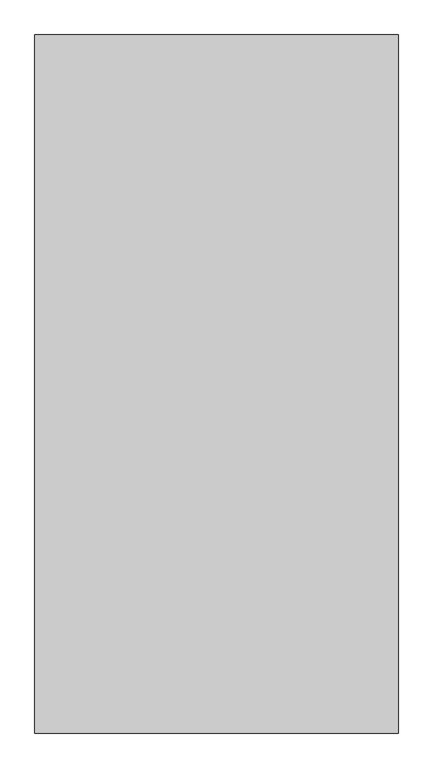
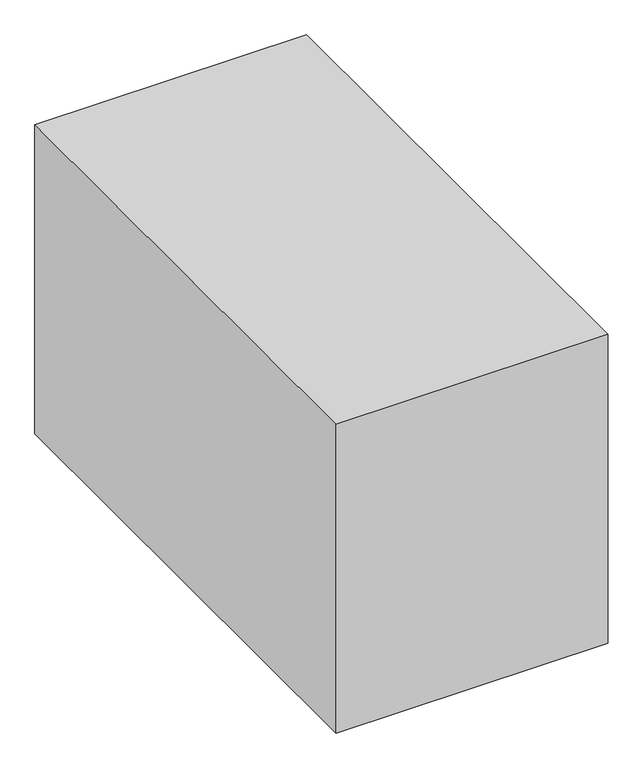
"""IFC4 building model written with IfcOpenShell, lengths in millimetres: proxy geometry, Space Planning Box_hec : Space Planning Box_hec."""

import ifcopenshell
import ifcopenshell.guid

model = None  # the IFC model being written
_history = None  # IfcOwnerHistory: only IFC2X3 demands one
_inside = {}  # id of a spatial element -> (the spatial element, [elements in it])
_under = {}  # id of a project, library or spatial element -> (it, [spatial elements below it])
_declared = {}  # id of a project -> (the project, [libraries it declares])
_typed = {}  # id of a type object -> (the type object, [elements of that type])
_made_of = {}  # id of a material, layer set ... -> (it, [elements and type objects made of it])


def new_model(schema):
    """Start an empty IFC model of exactly this schema.

    Asked for "IFC4X3", IfcOpenShell would pick the latest addendum, in which some entities
    have other attributes; the version numbers below select the first issue.
    IFC2X3 requires an IfcOwnerHistory on every rooted entity: one is made here for all.
    """
    global model, _history
    if schema == "IFC4X3":
        model = ifcopenshell.file(schema_version=(4, 3, 0, 0))
    else:
        model = ifcopenshell.file(schema=schema)
    _inside.clear()
    _under.clear()
    _declared.clear()
    _typed.clear()
    _made_of.clear()
    _history = None
    if model.schema == "IFC2X3":
        org = make("IfcOrganization", Name="unknown")
        user = make(
            "IfcPersonAndOrganization",
            ThePerson=make("IfcPerson", FamilyName="unknown"),
            TheOrganization=org,
        )
        app = make(
            "IfcApplication",
            ApplicationDeveloper=org,
            Version="unknown",
            ApplicationFullName="unknown",
            ApplicationIdentifier="unknown",
        )
        _history = make(
            "IfcOwnerHistory",
            OwningUser=user,
            OwningApplication=app,
            ChangeAction="ADDED",
            CreationDate=0,
        )
    return model


def make(cls, **values):
    """One entity of the class cls with the attributes given. An attribute that is None is left unset."""
    return model.create_entity(
        cls, **{name: value for name, value in values.items() if value is not None}
    )


def rooted(cls, **values):
    """An entity with a GlobalId (a new one), such as an element, a storey or a relation."""
    return make(cls, GlobalId=ifcopenshell.guid.new(), OwnerHistory=_history, **values)


def si_unit(unit_type, name, prefix=None):
    """IfcSIUnit, for example si_unit("LENGTHUNIT", "METRE", prefix="MILLI")."""
    return make("IfcSIUnit", UnitType=unit_type, Prefix=prefix, Name=name)


def assignment(units):
    """IfcUnitAssignment: the units of a project."""
    return None if units is None else make("IfcUnitAssignment", Units=units)


def point(xyz):
    """IfcCartesianPoint."""
    return None if xyz is None else make("IfcCartesianPoint", Coordinates=xyz)


def direction(xyz):
    """IfcDirection."""
    return None if xyz is None else make("IfcDirection", DirectionRatios=xyz)


def frame(location, z_axis=None, x_axis=None):
    """IfcAxis2Placement3D, a coordinate frame: its origin and axes. An axis left out is left unset."""
    return make(
        "IfcAxis2Placement3D",
        Location=point(location),
        Axis=direction(z_axis),
        RefDirection=direction(x_axis),
    )


def origin():
    """The frame at (0, 0, 0) with its axes left unset."""
    return frame((0.0, 0.0, 0.0))


def origin_with_axes():
    """The frame at (0, 0, 0) with the z axis (0, 0, 1) and the x axis (1, 0, 0) written out."""
    return frame((0.0, 0.0, 0.0), z_axis=(0.0, 0.0, 1.0), x_axis=(1.0, 0.0, 0.0))


def place(relative_to, where):
    """IfcLocalPlacement: puts the frame where relative to a parent placement (None: the world)."""
    return make(
        "IfcLocalPlacement", PlacementRelTo=relative_to, RelativePlacement=where
    )


def context(
    kind, dimensions, precision=None, world=None, true_north=None, identifier=None
):
    """IfcGeometricRepresentationContext, for example the 3D "Model" context."""
    return make(
        "IfcGeometricRepresentationContext",
        ContextIdentifier=identifier,
        ContextType=kind,
        CoordinateSpaceDimension=dimensions,
        Precision=precision,
        WorldCoordinateSystem=world,
        TrueNorth=true_north,
    )


def project(units=None, contexts=None):
    """IfcProject with its units and contexts."""
    return rooted(
        "IfcProject",
        Name="project",
        RepresentationContexts=contexts,
        UnitsInContext=assignment(units),
    )


def spatial(cls, under=None, at=None, **own):
    """A site, building, storey or space (cls), placed at a placement, below another one or the project."""
    s = rooted(cls, ObjectPlacement=at, **own)
    if under is not None:
        _under.setdefault(under.id(), (under, []))[1].append(s)
    return s


def polyline(points):
    """IfcPolyline through the points."""
    return make("IfcPolyline", Points=[point(p) for p in points])


def outline(outer, holes=None, kind="AREA"):
    """IfcArbitraryClosedProfileDef: a profile drawn as a closed curve; with holes, ...WithVoids."""
    if holes is None:
        return make("IfcArbitraryClosedProfileDef", ProfileType=kind, OuterCurve=outer)
    return make(
        "IfcArbitraryProfileDefWithVoids",
        ProfileType=kind,
        OuterCurve=outer,
        InnerCurves=holes,
    )


def extrude(swept, where, along, depth):
    """IfcExtrudedAreaSolid: the profile swept, set in the frame where, extruded along a direction by depth."""
    return make(
        "IfcExtrudedAreaSolid",
        SweptArea=swept,
        Position=where,
        ExtrudedDirection=direction(along),
        Depth=depth,
    )


def shape(context_of_items, identifier, shape_type, items):
    """IfcShapeRepresentation: the items that make up one representation, for example the "Body"."""
    return make(
        "IfcShapeRepresentation",
        ContextOfItems=context_of_items,
        RepresentationIdentifier=identifier,
        RepresentationType=shape_type,
        Items=items,
    )


def source(mapping_origin, context_of_items, identifier, shape_type, items):
    """IfcRepresentationMap: a shape defined once, which mapped items show again and again."""
    return make(
        "IfcRepresentationMap",
        MappingOrigin=mapping_origin,
        MappedRepresentation=shape(context_of_items, identifier, shape_type, items),
    )


def transform(
    local_origin,
    x_axis=None,
    y_axis=None,
    z_axis=None,
    scale=None,
    scale2=None,
    scale3=None,
    uniform=True,
):
    """IfcCartesianTransformationOperator3D, or its non-uniform kind. x_axis, y_axis, z_axis: its Axis1, 2, 3."""
    if uniform:
        return make(
            "IfcCartesianTransformationOperator3D",
            Axis1=direction(x_axis),
            Axis2=direction(y_axis),
            LocalOrigin=point(local_origin),
            Scale=scale,
            Axis3=direction(z_axis),
        )
    return make(
        "IfcCartesianTransformationOperator3DnonUniform",
        Axis1=direction(x_axis),
        Axis2=direction(y_axis),
        LocalOrigin=point(local_origin),
        Scale=scale,
        Axis3=direction(z_axis),
        Scale2=scale2,
        Scale3=scale3,
    )


def mapped(mapping_source, mapping_target):
    """IfcMappedItem: shows the shape of a source again, moved by a transform."""
    return make(
        "IfcMappedItem", MappingSource=mapping_source, MappingTarget=mapping_target
    )


def made_of(thing, what):
    """Note that an element or type object is made of a material, layer set ...; save() writes the relation."""
    if what is not None:
        _made_of.setdefault(what.id(), (what, []))[1].append(thing)
    return thing


def element(
    cls,
    number,
    at=None,
    inside=None,
    cuts=None,
    type_object=None,
    material=None,
    context=None,
    identifier="Body",
    shape_type=None,
    held_by="IfcProductDefinitionShape",
    body=None,
    shapes=None,
    **own,
):
    """One element of the class cls, such as IfcWall. Its Tag is "e" and its number.

    at: its placement. inside: the storey or other place that contains it. cuts: it is an
    opening in that element (IfcRelVoidsElement). A single representation is given by context,
    identifier, shape_type and body (its items); several are given by shapes. held_by: the class
    of the entity that holds the representations. save() writes the other relations.
    """
    e = rooted(cls, Tag="e%d" % number, ObjectPlacement=at, **own)
    if body is not None:
        shapes = [shape(context, identifier, shape_type, body)]
    if shapes is not None:
        e.Representation = make(held_by, Representations=shapes)
    if inside is not None:
        _inside.setdefault(inside.id(), (inside, []))[1].append(e)
    if cuts is not None:
        rooted(
            "IfcRelVoidsElement", RelatingBuildingElement=cuts, RelatedOpeningElement=e
        )
    if type_object is not None:
        _typed.setdefault(type_object.id(), (type_object, []))[1].append(e)
    return made_of(e, material)


def aggregate(whole, parts):
    """IfcRelAggregates: a whole, such as a stair, and the parts it consists of."""
    return rooted("IfcRelAggregates", RelatingObject=whole, RelatedObjects=parts)


def save(model, path):
    """Write the relations noted so far, then the file.

    IfcRelAggregates (storeys below a building ...), IfcRelContainedInSpatialStructure (elements
    in a storey), IfcRelDefinesByType, IfcRelAssociatesMaterial and IfcRelDeclares: one each for
    every whole, place, type object, material and project.
    """
    for whole, parts in _under.values():
        aggregate(whole, parts)
    for where, things in _inside.values():
        rooted(
            "IfcRelContainedInSpatialStructure",
            RelatedElements=things,
            RelatingStructure=where,
        )
    for kind, things in _typed.values():
        rooted("IfcRelDefinesByType", RelatedObjects=things, RelatingType=kind)
    for what, things in _made_of.values():
        rooted("IfcRelAssociatesMaterial", RelatedObjects=things, RelatingMaterial=what)
    for by, libraries in _declared.values():
        rooted("IfcRelDeclares", RelatingContext=by, RelatedDefinitions=libraries)
    model.write(path)


def generic_models_7902148a(model_context):
    return source(origin(), model_context, "Body", "SweptSolid", [
        extrude(outline(polyline([(2500.0, 4800.0), (2500.0, -4800.0), (-2500.0, -4800.0), (-2500.0, 4800.0), (2500.0, 4800.0)])), origin_with_axes(), (0.0, 0.0, 1.0), 6000.0),
    ])


if __name__ == "__main__":
    model = new_model("IFC4")
    model_context = context("Model", 3, world=origin())
    ifc_project = project(units=[si_unit("LENGTHUNIT", "METRE", prefix="MILLI")], contexts=[model_context])
    site = spatial("IfcSite", under=ifc_project)
    building = spatial("IfcBuilding", under=site)
    placement = place(None, origin())
    generic_models_shape = generic_models_7902148a(model_context)
    element("IfcBuildingElementProxy", 1, Name="Space Planning Box_hec : Space Planning Box_hec", ObjectType="Space Planning Box_hec : Space Planning Box_hec", at=placement, inside=building, context=model_context, shape_type="MappedRepresentation", body=[
        mapped(generic_models_shape, transform((0.0, 0.0, 0.0), x_axis=(1.0, 0.0, 0.0), y_axis=(0.0, 1.0, 0.0), z_axis=(0.0, 0.0, 1.0))),
    ])
    save(model, "model.ifc")

# Revit data of these elements
# Type "Space Planning Box_hec : Space Planning Box_hec"
#   Type Comments = "..."
#   Room Name [instance default] = "?"
#   Interior Finish [instance default] = ""
#   Exterior Finish [instance default] = ""
#   Department [instance default] = ""
#   Assembly Code = "..."
#   Width [instance default] = 1524 mm
#   Program Area [instance default] = 0.00 m²
#   Length [instance default] = 1524 mm
#   Height [instance default] = 1524 mm
#   Area [instance default] = 2.32258 m²
#   Fill Color [instance default] = Cyan
#   Default Elevation = 0
# Element 1 (IfcBuildingElementProxy, "Space Planning Box_hec : Space Planning Box_hec")
#   Room Name = "Document Room"
#   Interior Finish = "IF2-1"
#   Exterior Finish = "EF1"
#   Department = "AR"
#   Width = 5000 mm
#   Program Area = 48.00 m²
#   Length = 9600 mm
#   Height = 6000 mm
#   Area = 48.00 m²
#   Fill Color = Lavender
#   Materials on its faces: "Lavender"
# Materials
#   "Cyan": class "Generic", colour RGB 0 255 255, transparency 0.2, Cost = 0
#   "Lavender": class "Generic", colour RGB 186 85 211, transparency 0.2, Cost = 0
